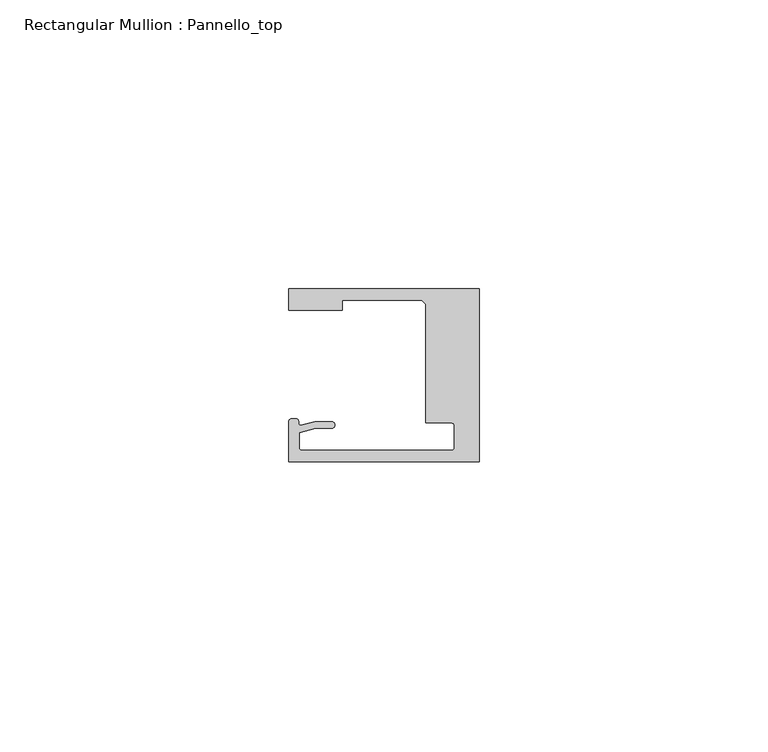
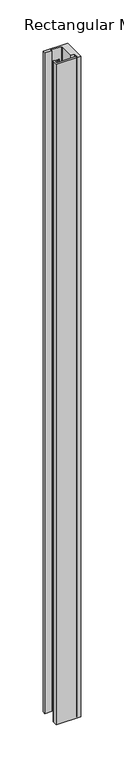
"""IFC4 building model written with IfcOpenShell, lengths in millimetres: member geometry, Rectangular Mullion : Pannello_top."""

from ifc_helpers import new_model, si_unit, frame, origin, place, context, project, spatial, polyline, circle_curve, source, transform, mapped, element, save
from ifc_brep_helpers import plane_surface, cylinder_surface, revolved_surface, extruded_surface, spline_curve, advanced_brep


def rectangular_mullion_pannello_top_b0e7c652(model_context):
    return source(origin(), model_context, "Body", "AdvancedBrep", [
        advanced_brep(
        [(-33.0, 15.0, 0.0), (-33.0, 11.3000004, 0.0), (-23.700041, 11.3000004, 0.0), (-23.700041, 13.0000004, 0.0), (-10.0000103, 13.0000004, 0.0), (-9.2999726, 12.2999849, 0.0), (-9.2999726, -8.2500595, 0.0), (-4.7999726, -8.2500595, 0.0), (-4.2999726, -8.7500595, 0.0), (-4.2999726, -12.50001, 0.0), (-4.7999726, -13.00001, 0.0), (-30.69998, -13.00001, 0.0), (-31.19998, -12.50001, 0.0), (-31.19998, -9.9657591, 0.0), (-28.3419477, -9.1999523, 0.0), (-25.59998, -9.1999523, 0.0), (-25.59998, -7.9999523, 0.0), (-28.4999305, -7.9999523, 0.0), (-30.9223017, -8.6490241, 0.0), (-33.0000135, -8.0000472, 0.0), (-33.0000135, -15.0, 0.0), (0.0, -15.0, 0.0), (0.0, 15.0, 0.0), (-33.0, 15.0, -933.9999729), (0.0, 15.0, -933.9999729), (0.0, -15.0, -933.9999729), (-33.0000135, -15.0, -933.9999729), (-33.0000135, -8.0000472, -933.9999729), (-30.9223017, -8.6490241, -933.9999729), (-28.4999305, -7.9999523, -933.9999729), (-25.59998, -7.9999523, -933.9999729), (-25.59998, -9.1999523, -933.9999729), (-28.3419477, -9.1999523, -933.9999729), (-31.19998, -9.9657591, -933.9999729), (-31.19998, -12.50001, -933.9999729), (-30.69998, -13.00001, -933.9999729), (-4.7999726, -13.00001, -933.9999729), (-4.2999726, -12.50001, -933.9999729), (-4.2999726, -8.7500595, -933.9999729), (-4.7999726, -8.2500595, -933.9999729), (-9.2999726, -8.2500595, -933.9999729), (-9.2999726, 12.2999849, -933.9999729), (-10.0000103, 13.0000004, -933.9999729), (-23.700041, 13.0000004, -933.9999729), (-23.700041, 11.3000004, -933.9999729), (-33.0, 11.3000004, -933.9999729)],
        [
            (0, 1),
            (1, 2),
            (2, 3),
            (3, 4),
            (4, 5),
            (5, 6),
            (6, 7),
            (7, 8, circle_curve(frame((-4.7999726, -8.7500595, 0.0), z_axis=(0.0, 0.0, -1.0), x_axis=(0.0, 1.0, 0.0)), 0.5)),
            (8, 9),
            (9, 10, circle_curve(frame((-4.7999726, -12.50001, 0.0), z_axis=(0.0, 0.0, -1.0), x_axis=(1.0, 0.0, 0.0)), 0.5)),
            (10, 11),
            (11, 12, circle_curve(frame((-30.69998, -12.50001, 0.0), z_axis=(0.0, 0.0, -1.0), x_axis=(0.0, -1.0, 0.0)), 0.5)),
            (12, 13),
            (13, 14),
            (14, 15),
            (15, 16, circle_curve(frame((-25.59998, -8.5999523, 0.0), z_axis=(0.0, 0.0, 1.0), x_axis=(0.0, -1.0, 0.0)), 0.6)),
            (16, 17),
            (17, 18),
            (18, 19, spline_curve(3, [(-30.9223017, -8.6490241, 0.0), (-31.312054066, -8.717747958, 0.0), (-31.298563602, -8.366228555, 0.0), (-31.305645054, -7.690065204, 0.0), (-31.357433266, -7.563996614, 0.0), (-32.262327879, -7.456527435, 0.0), (-33.0000135, -7.457047519, 0.0), (-33.0000135, -8.0000472, 0.0)], [4, 2, 2, 4], [0.0, 0.001840817752199412, 0.004996616814974408, 0.007702013405570312])),
            (19, 20),
            (20, 21),
            (21, 22),
            (22, 0),
            (23, 24),
            (24, 25),
            (25, 26),
            (26, 27),
            (27, 28, spline_curve(3, [(-33.0000135, -8.0000472, -933.9999729), (-33.0000135, -7.457047519, -933.9999729), (-32.262327879, -7.456527435, -933.9999729), (-31.357433266, -7.563996614, -933.9999729), (-31.305645054, -7.690065204, -933.9999729), (-31.298563602, -8.366228555, -933.9999729), (-31.312054066, -8.717747958, -933.9999729), (-30.9223017, -8.6490241, -933.9999729)], [4, 2, 2, 4], [0.0, 0.0027053965905959043, 0.0058611956533709, 0.007702013405570312])),
            (28, 29),
            (29, 30),
            (30, 31, circle_curve(frame((-25.59998, -8.5999523, -933.9999729), z_axis=(0.0, 0.0, -1.0), x_axis=(0.0, -1.0, 0.0)), 0.6)),
            (31, 32),
            (32, 33),
            (33, 34),
            (34, 35, circle_curve(frame((-30.69998, -12.50001, -933.9999729), z_axis=(0.0, 0.0, 1.0), x_axis=(0.0, -1.0, 0.0)), 0.5)),
            (35, 36),
            (36, 37, circle_curve(frame((-4.7999726, -12.50001, -933.9999729), z_axis=(0.0, 0.0, 1.0), x_axis=(1.0, 0.0, 0.0)), 0.5)),
            (37, 38),
            (38, 39, circle_curve(frame((-4.7999726, -8.7500595, -933.9999729), z_axis=(0.0, 0.0, 1.0), x_axis=(0.0, 1.0, 0.0)), 0.5)),
            (39, 40),
            (40, 41),
            (41, 42),
            (42, 43),
            (43, 44),
            (44, 45),
            (45, 23),
            (0, 23),
            (45, 1),
            (44, 2),
            (43, 3),
            (42, 4),
            (41, 5),
            (40, 6),
            (39, 7),
            (38, 8),
            (37, 9),
            (36, 10),
            (35, 11),
            (34, 12),
            (33, 13),
            (32, 14),
            (31, 15),
            (30, 16),
            (29, 17),
            (28, 18),
            (27, 19),
            (26, 20),
            (25, 21),
            (24, 22),
        ],
        [
            plane_surface(frame((0.0, -36.2491502, 0.0), z_axis=(0.0, 0.0, 1.0), x_axis=(-1.0, 0.0, 0.0))),
            plane_surface(frame((0.0, -36.2491502, -933.9999729), z_axis=(0.0, 0.0, -1.0), x_axis=(-1.0, 0.0, 0.0))),
            plane_surface(frame((-33.0, 15.0, 0.0), z_axis=(-1.0, 0.0, 0.0), x_axis=(0.0, 0.0, -1.0))),
            plane_surface(frame((-33.0, 11.3000004, 0.0), z_axis=(0.0, -1.0, 0.0), x_axis=(0.0, 0.0, -1.0))),
            plane_surface(frame((-23.700041, 11.3000004, 0.0), z_axis=(1.0, 0.0, 0.0), x_axis=(0.0, 0.0, -1.0))),
            plane_surface(frame((-23.700041, 13.0000004, 0.0), z_axis=(0.0, -1.0, 0.0), x_axis=(0.0, 0.0, -1.0))),
            plane_surface(frame((-10.0000103, 13.0000004, 0.0), z_axis=(-0.7070955486277984, -0.7071180135668678, 0.0), x_axis=(0.0, 0.0, -1.0))),
            plane_surface(frame((-9.2999726, 12.2999849, 0.0), z_axis=(-1.0, 0.0, 0.0), x_axis=(0.0, 0.0, -1.0))),
            plane_surface(frame((-9.2999726, -8.2500595, 0.0), z_axis=(0.0, -1.0, 0.0), x_axis=(0.0, 0.0, -1.0))),
            revolved_surface(polyline([(-4.7999726, -8.2500595, -933.9999729), (-4.7999726, -8.2500595, 0.0)]), (-4.7999726, -8.7500595, 0.0), (0.0, 0.0, -1.0)),
            plane_surface(frame((-4.2999726, -8.7500595, 0.0), z_axis=(-1.0, 0.0, 0.0), x_axis=(0.0, 0.0, -1.0))),
            revolved_surface(polyline([(-4.2999726, -12.50001, -933.9999729), (-4.2999726, -12.50001, 0.0)]), (-4.7999726, -12.50001, 0.0), (0.0, 0.0, -1.0)),
            plane_surface(frame((-4.7999726, -13.00001, 0.0), z_axis=(0.0, 1.0, 0.0), x_axis=(0.0, 0.0, -1.0))),
            revolved_surface(polyline([(-30.69998, -13.00001, -933.9999729), (-30.69998, -13.00001, 0.0)]), (-30.69998, -12.50001, 0.0), (0.0, 0.0, -1.0)),
            plane_surface(frame((-31.19998, -12.50001, 0.0), z_axis=(1.0, 0.0, 0.0), x_axis=(0.0, 0.0, -1.0))),
            plane_surface(frame((-31.19998, -9.9657591, 0.0), z_axis=(0.25881883204288636, -0.9659258833782002, 0.0), x_axis=(0.0, 0.0, -1.0))),
            plane_surface(frame((-28.3419477, -9.1999523, 0.0), z_axis=(0.0, -1.0, 0.0), x_axis=(0.0, 0.0, -1.0))),
            cylinder_surface(frame((-25.59998, -8.5999523, 0.0), z_axis=(0.0, 0.0, 1.0), x_axis=(0.0, -1.0, 0.0)), 0.6),
            plane_surface(frame((-25.59998, -7.9999523, 0.0), z_axis=(0.0, 1.0, 0.0), x_axis=(0.0, 0.0, -1.0))),
            plane_surface(frame((-28.4999305, -7.9999523, 0.0), z_axis=(-0.25881883200192934, 0.9659258833891746, 0.0), x_axis=(0.0, 0.0, -1.0))),
            extruded_surface(spline_curve(3, [(-30.9223017, -8.6490241, -933.9999729), (-31.312054066, -8.717747958, -933.9999729), (-31.298563602, -8.366228555, -933.9999729), (-31.305645054, -7.690065204, -933.9999729), (-31.357433266, -7.563996614, -933.9999729), (-32.262327879, -7.456527435, -933.9999729), (-33.0000135, -7.457047519, -933.9999729), (-33.0000135, -8.0000472, -933.9999729)], [4, 2, 2, 4], [0.0, 0.001840817752199412, 0.004996616814974408, 0.007702013405570312]), (0.0, 0.0, 933.9999729), 933.9999729),
            plane_surface(frame((-33.0000135, -8.0000472, 0.0), z_axis=(-1.0, 0.0, 0.0), x_axis=(0.0, 0.0, -1.0))),
            plane_surface(frame((-33.0000135, -15.0, 0.0), z_axis=(0.0, -1.0, 0.0), x_axis=(0.0, 0.0, -1.0))),
            plane_surface(frame((0.0, -15.0, 0.0), z_axis=(1.0, 0.0, 0.0), x_axis=(0.0, 0.0, -1.0))),
            plane_surface(frame((0.0, 15.0, 0.0), z_axis=(0.0, 1.0, 0.0), x_axis=(0.0, 0.0, -1.0))),
        ],
        [
            (0, [[1, 2, 3, 4, 5, 6, 7, 8, 9, 10, 11, 12, 13, 14, 15, 16, 17, 18, 19, 20, 21, 22, 23]]),
            (1, [[24, 25, 26, 27, 28, 29, 30, 31, 32, 33, 34, 35, 36, 37, 38, 39, 40, 41, 42, 43, 44, 45, 46]]),
            (2, [[-1, 47, -46, 48]]),
            (3, [[-2, -48, -45, 49]]),
            (4, [[-3, -49, -44, 50]]),
            (5, [[-4, -50, -43, 51]]),
            (6, [[-5, -51, -42, 52]]),
            (7, [[-6, -52, -41, 53]]),
            (8, [[-7, -53, -40, 54]]),
            (9, [[-8, -54, -39, 55]]),
            (10, [[-9, -55, -38, 56]]),
            (11, [[-10, -56, -37, 57]]),
            (12, [[-11, -57, -36, 58]]),
            (13, [[-12, -58, -35, 59]]),
            (14, [[-13, -59, -34, 60]]),
            (15, [[-14, -60, -33, 61]]),
            (16, [[-15, -61, -32, 62]]),
            (17, [[-16, -62, -31, 63]]),
            (18, [[-17, -63, -30, 64]]),
            (19, [[-18, -64, -29, 65]]),
            (20, [[-19, -65, -28, 66]]),
            (21, [[-20, -66, -27, 67]]),
            (22, [[-21, -67, -26, 68]]),
            (23, [[-22, -68, -25, 69]]),
            (24, [[-23, -69, -24, -47]]),
        ],
    ),
    ])


if __name__ == "__main__":
    model = new_model("IFC4")
    model_context = context("Model", 3, world=origin())
    ifc_project = project(units=[si_unit("LENGTHUNIT", "METRE", prefix="MILLI")], contexts=[model_context])
    site = spatial("IfcSite", under=ifc_project)
    building = spatial("IfcBuilding", under=site)
    placement = place(None, origin())
    rectangular_mullion_pannello_top_shape = rectangular_mullion_pannello_top_b0e7c652(model_context)
    element("IfcMember", 1, ObjectType="Rectangular Mullion : Pannello_top", at=placement, inside=building, context=model_context, shape_type="MappedRepresentation", body=[
        mapped(rectangular_mullion_pannello_top_shape, transform((0.0, 0.0, 0.0), x_axis=(1.0, 0.0, 0.0), y_axis=(0.0, 1.0, 0.0), z_axis=(0.0, 0.0, 1.0))),
    ])
    save(model, "model.ifc")

# Revit data of these elements
# Type "Rectangular Mullion : Pannello_top"
#   built-in parameter 1007322 = 0.0984252 (stored number, unit not read)
#   built-in parameter 1007321 = 0 (stored number, unit not read)
#   built-in parameter 1007320 = 0.0305117 (stored number, unit not read)
